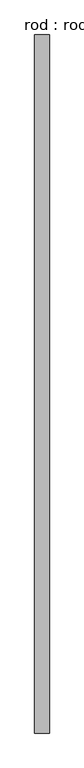
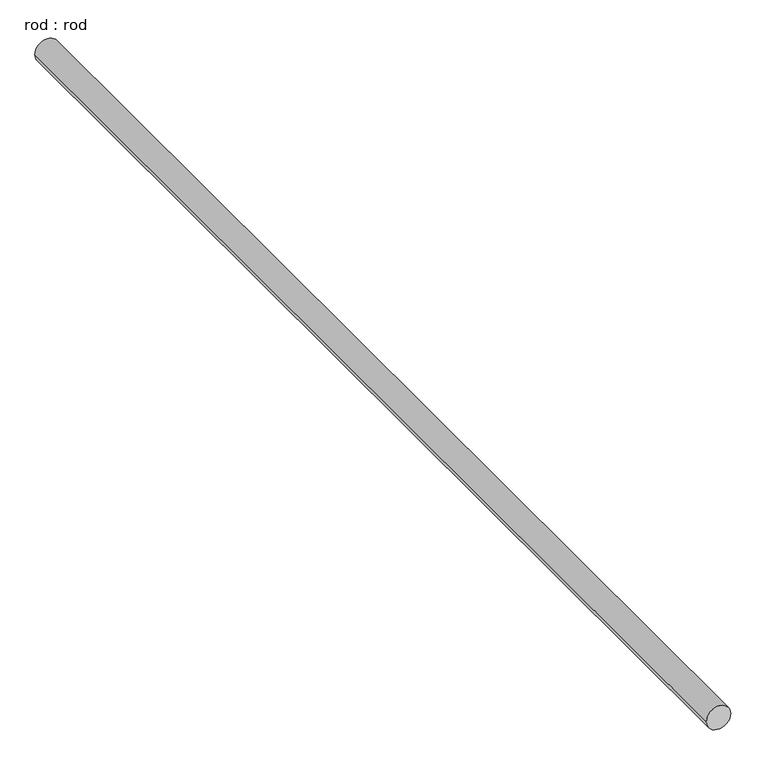
"""IFC4 building model written with IfcOpenShell, lengths in millimetres: proxy geometry, rod : rod."""

from ifc_helpers import new_model, si_unit, point, frame, frame_2d, origin, place, context, project, spatial, circle_curve, trimmed, segment, composite_curve, outline, extrude, source, transform, mapped, element, save


def rod_rod_95733b82(model_context):
    return source(origin(), model_context, "Body", "SweptSolid", [
        extrude(outline(composite_curve([segment(trimmed(circle_curve(frame_2d((0.0108462, 0.0)), 200.0), [point((0.0108462, 200.0))], [point((0.0108462, -200.0))], False, "CARTESIAN"), True, "CONTINUOUS"), segment(trimmed(circle_curve(frame_2d((0.0108462, 0.0)), 200.0), [point((0.0108462, -200.0))], [point((0.0108462, 200.0))], False, "CARTESIAN"), True, "CONTINUOUS")], self_intersect=False)), frame((0.0, -5444.8942541, 0.0), z_axis=(0.0, 1.0, 0.0), x_axis=(0.0, 0.0, 1.0)), (0.0, 0.0, 1.0), 19075.2457389),
    ])


if __name__ == "__main__":
    model = new_model("IFC4")
    model_context = context("Model", 3, world=origin())
    ifc_project = project(units=[si_unit("LENGTHUNIT", "METRE", prefix="MILLI")], contexts=[model_context])
    site = spatial("IfcSite", under=ifc_project)
    building = spatial("IfcBuilding", under=site)
    placement = place(None, origin())
    rod_rod_shape = rod_rod_95733b82(model_context)
    element("IfcBuildingElementProxy", 1, Name="rod : rod", ObjectType="rod : rod", at=placement, inside=building, context=model_context, shape_type="MappedRepresentation", body=[
        mapped(rod_rod_shape, transform((0.0, 0.0, 0.0), x_axis=(1.0, 0.0, 0.0), y_axis=(0.0, 1.0, 0.0), z_axis=(0.0, 0.0, 1.0))),
    ])
    save(model, "model.ifc")

# Revit data of these elements
# Type "rod : rod"
#   Default Elevation = 0
